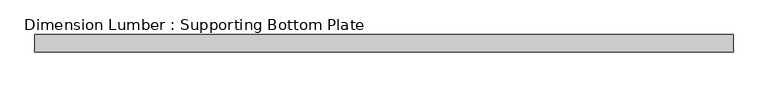
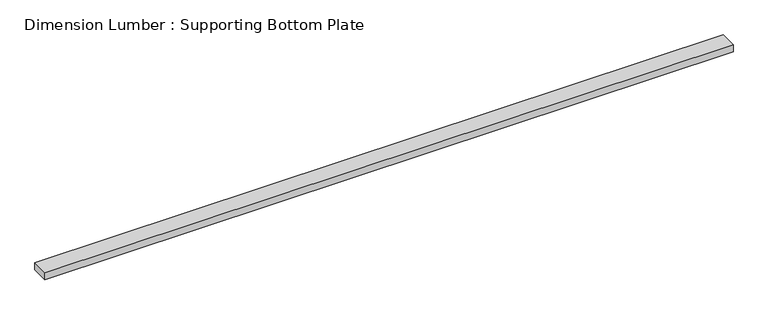
"""IFC4 building model written with IfcOpenShell, lengths in millimetres: beam geometry, Dimension Lumber : Supporting Bottom Plate."""

import ifcopenshell
import ifcopenshell.guid

model = None  # the IFC model being written
_history = None  # IfcOwnerHistory: only IFC2X3 demands one
_inside = {}  # id of a spatial element -> (the spatial element, [elements in it])
_under = {}  # id of a project, library or spatial element -> (it, [spatial elements below it])
_declared = {}  # id of a project -> (the project, [libraries it declares])
_typed = {}  # id of a type object -> (the type object, [elements of that type])
_made_of = {}  # id of a material, layer set ... -> (it, [elements and type objects made of it])


def new_model(schema):
    """Start an empty IFC model of exactly this schema.

    Asked for "IFC4X3", IfcOpenShell would pick the latest addendum, in which some entities
    have other attributes; the version numbers below select the first issue.
    IFC2X3 requires an IfcOwnerHistory on every rooted entity: one is made here for all.
    """
    global model, _history
    if schema == "IFC4X3":
        model = ifcopenshell.file(schema_version=(4, 3, 0, 0))
    else:
        model = ifcopenshell.file(schema=schema)
    _inside.clear()
    _under.clear()
    _declared.clear()
    _typed.clear()
    _made_of.clear()
    _history = None
    if model.schema == "IFC2X3":
        org = make("IfcOrganization", Name="unknown")
        user = make(
            "IfcPersonAndOrganization",
            ThePerson=make("IfcPerson", FamilyName="unknown"),
            TheOrganization=org,
        )
        app = make(
            "IfcApplication",
            ApplicationDeveloper=org,
            Version="unknown",
            ApplicationFullName="unknown",
            ApplicationIdentifier="unknown",
        )
        _history = make(
            "IfcOwnerHistory",
            OwningUser=user,
            OwningApplication=app,
            ChangeAction="ADDED",
            CreationDate=0,
        )
    return model


def make(cls, **values):
    """One entity of the class cls with the attributes given. An attribute that is None is left unset."""
    return model.create_entity(
        cls, **{name: value for name, value in values.items() if value is not None}
    )


def rooted(cls, **values):
    """An entity with a GlobalId (a new one), such as an element, a storey or a relation."""
    return make(cls, GlobalId=ifcopenshell.guid.new(), OwnerHistory=_history, **values)


def si_unit(unit_type, name, prefix=None):
    """IfcSIUnit, for example si_unit("LENGTHUNIT", "METRE", prefix="MILLI")."""
    return make("IfcSIUnit", UnitType=unit_type, Prefix=prefix, Name=name)


def assignment(units):
    """IfcUnitAssignment: the units of a project."""
    return None if units is None else make("IfcUnitAssignment", Units=units)


def point(xyz):
    """IfcCartesianPoint."""
    return None if xyz is None else make("IfcCartesianPoint", Coordinates=xyz)


def direction(xyz):
    """IfcDirection."""
    return None if xyz is None else make("IfcDirection", DirectionRatios=xyz)


def frame(location, z_axis=None, x_axis=None):
    """IfcAxis2Placement3D, a coordinate frame: its origin and axes. An axis left out is left unset."""
    return make(
        "IfcAxis2Placement3D",
        Location=point(location),
        Axis=direction(z_axis),
        RefDirection=direction(x_axis),
    )


def origin():
    """The frame at (0, 0, 0) with its axes left unset."""
    return frame((0.0, 0.0, 0.0))


def place(relative_to, where):
    """IfcLocalPlacement: puts the frame where relative to a parent placement (None: the world)."""
    return make(
        "IfcLocalPlacement", PlacementRelTo=relative_to, RelativePlacement=where
    )


def context(
    kind, dimensions, precision=None, world=None, true_north=None, identifier=None
):
    """IfcGeometricRepresentationContext, for example the 3D "Model" context."""
    return make(
        "IfcGeometricRepresentationContext",
        ContextIdentifier=identifier,
        ContextType=kind,
        CoordinateSpaceDimension=dimensions,
        Precision=precision,
        WorldCoordinateSystem=world,
        TrueNorth=true_north,
    )


def project(units=None, contexts=None):
    """IfcProject with its units and contexts."""
    return rooted(
        "IfcProject",
        Name="project",
        RepresentationContexts=contexts,
        UnitsInContext=assignment(units),
    )


def spatial(cls, under=None, at=None, **own):
    """A site, building, storey or space (cls), placed at a placement, below another one or the project."""
    s = rooted(cls, ObjectPlacement=at, **own)
    if under is not None:
        _under.setdefault(under.id(), (under, []))[1].append(s)
    return s


def polyline(points):
    """IfcPolyline through the points."""
    return make("IfcPolyline", Points=[point(p) for p in points])


def outline(outer, holes=None, kind="AREA"):
    """IfcArbitraryClosedProfileDef: a profile drawn as a closed curve; with holes, ...WithVoids."""
    if holes is None:
        return make("IfcArbitraryClosedProfileDef", ProfileType=kind, OuterCurve=outer)
    return make(
        "IfcArbitraryProfileDefWithVoids",
        ProfileType=kind,
        OuterCurve=outer,
        InnerCurves=holes,
    )


def extrude(swept, where, along, depth):
    """IfcExtrudedAreaSolid: the profile swept, set in the frame where, extruded along a direction by depth."""
    return make(
        "IfcExtrudedAreaSolid",
        SweptArea=swept,
        Position=where,
        ExtrudedDirection=direction(along),
        Depth=depth,
    )


def shape(context_of_items, identifier, shape_type, items):
    """IfcShapeRepresentation: the items that make up one representation, for example the "Body"."""
    return make(
        "IfcShapeRepresentation",
        ContextOfItems=context_of_items,
        RepresentationIdentifier=identifier,
        RepresentationType=shape_type,
        Items=items,
    )


def source(mapping_origin, context_of_items, identifier, shape_type, items):
    """IfcRepresentationMap: a shape defined once, which mapped items show again and again."""
    return make(
        "IfcRepresentationMap",
        MappingOrigin=mapping_origin,
        MappedRepresentation=shape(context_of_items, identifier, shape_type, items),
    )


def transform(
    local_origin,
    x_axis=None,
    y_axis=None,
    z_axis=None,
    scale=None,
    scale2=None,
    scale3=None,
    uniform=True,
):
    """IfcCartesianTransformationOperator3D, or its non-uniform kind. x_axis, y_axis, z_axis: its Axis1, 2, 3."""
    if uniform:
        return make(
            "IfcCartesianTransformationOperator3D",
            Axis1=direction(x_axis),
            Axis2=direction(y_axis),
            LocalOrigin=point(local_origin),
            Scale=scale,
            Axis3=direction(z_axis),
        )
    return make(
        "IfcCartesianTransformationOperator3DnonUniform",
        Axis1=direction(x_axis),
        Axis2=direction(y_axis),
        LocalOrigin=point(local_origin),
        Scale=scale,
        Axis3=direction(z_axis),
        Scale2=scale2,
        Scale3=scale3,
    )


def mapped(mapping_source, mapping_target):
    """IfcMappedItem: shows the shape of a source again, moved by a transform."""
    return make(
        "IfcMappedItem", MappingSource=mapping_source, MappingTarget=mapping_target
    )


def made_of(thing, what):
    """Note that an element or type object is made of a material, layer set ...; save() writes the relation."""
    if what is not None:
        _made_of.setdefault(what.id(), (what, []))[1].append(thing)
    return thing


def element(
    cls,
    number,
    at=None,
    inside=None,
    cuts=None,
    type_object=None,
    material=None,
    context=None,
    identifier="Body",
    shape_type=None,
    held_by="IfcProductDefinitionShape",
    body=None,
    shapes=None,
    **own,
):
    """One element of the class cls, such as IfcWall. Its Tag is "e" and its number.

    at: its placement. inside: the storey or other place that contains it. cuts: it is an
    opening in that element (IfcRelVoidsElement). A single representation is given by context,
    identifier, shape_type and body (its items); several are given by shapes. held_by: the class
    of the entity that holds the representations. save() writes the other relations.
    """
    e = rooted(cls, Tag="e%d" % number, ObjectPlacement=at, **own)
    if body is not None:
        shapes = [shape(context, identifier, shape_type, body)]
    if shapes is not None:
        e.Representation = make(held_by, Representations=shapes)
    if inside is not None:
        _inside.setdefault(inside.id(), (inside, []))[1].append(e)
    if cuts is not None:
        rooted(
            "IfcRelVoidsElement", RelatingBuildingElement=cuts, RelatedOpeningElement=e
        )
    if type_object is not None:
        _typed.setdefault(type_object.id(), (type_object, []))[1].append(e)
    return made_of(e, material)


def aggregate(whole, parts):
    """IfcRelAggregates: a whole, such as a stair, and the parts it consists of."""
    return rooted("IfcRelAggregates", RelatingObject=whole, RelatedObjects=parts)


def save(model, path):
    """Write the relations noted so far, then the file.

    IfcRelAggregates (storeys below a building ...), IfcRelContainedInSpatialStructure (elements
    in a storey), IfcRelDefinesByType, IfcRelAssociatesMaterial and IfcRelDeclares: one each for
    every whole, place, type object, material and project.
    """
    for whole, parts in _under.values():
        aggregate(whole, parts)
    for where, things in _inside.values():
        rooted(
            "IfcRelContainedInSpatialStructure",
            RelatedElements=things,
            RelatingStructure=where,
        )
    for kind, things in _typed.values():
        rooted("IfcRelDefinesByType", RelatedObjects=things, RelatingType=kind)
    for what, things in _made_of.values():
        rooted("IfcRelAssociatesMaterial", RelatedObjects=things, RelatingMaterial=what)
    for by, libraries in _declared.values():
        rooted("IfcRelDeclares", RelatingContext=by, RelatedDefinitions=libraries)
    model.write(path)


def dimension_lumber_supporting_bottom_plate_2ddee0ef(model_context):
    return source(origin(), model_context, "Body", "SweptSolid", [
        extrude(outline(polyline([(1771.65, 44.45), (1771.65, -44.45), (-1768.475, -44.45), (-1768.475, 44.45), (1771.65, 44.45)])), frame((0.0, 0.0, -19.05), z_axis=(0.0, 0.0, 1.0), x_axis=(1.0, 0.0, 0.0)), (0.0, 0.0, 1.0), 38.1),
    ])


if __name__ == "__main__":
    model = new_model("IFC4")
    model_context = context("Model", 3, world=origin())
    ifc_project = project(units=[si_unit("LENGTHUNIT", "METRE", prefix="MILLI")], contexts=[model_context])
    site = spatial("IfcSite", under=ifc_project)
    building = spatial("IfcBuilding", under=site)
    placement = place(None, origin())
    dimension_lumber_supporting_bottom_plate_shape = dimension_lumber_supporting_bottom_plate_2ddee0ef(model_context)
    element("IfcBeam", 1, ObjectType="Dimension Lumber : Supporting Bottom Plate", at=placement, inside=building, context=model_context, shape_type="MappedRepresentation", body=[
        mapped(dimension_lumber_supporting_bottom_plate_shape, transform((0.0, 0.0, 0.0), x_axis=(1.0, 0.0, 0.0), y_axis=(0.0, 1.0, 0.0), z_axis=(0.0, 0.0, 1.0))),
    ])
    save(model, "model.ifc")

# Revit data of these elements
# Type "Dimension Lumber : Supporting Bottom Plate"
#   Assembly Code = "B10"
#   A = 0.0364583 SF
#   Length [instance default] = 5' - 0"
#   b = 0' - 3 1/2"
#   d = 0' - 1 1/2"
#   Structural Material [instance default] = Softwood, Lumber
# Element 1 (IfcBeam, "Dimension Lumber : Supporting Bottom Plate")
#   Structural Material = Douglas Fir #2
#   Materials on its faces: "Douglas Fir #2"
# Materials
#   "Softwood, Lumber": class "Wood", colour RGB 223 192 134, transparency 0, Description = "Pinus Echinata", Cost = 0
#   "Douglas Fir #2": class "Wood", colour RGB 223 192 134, transparency 0, Description = "Pinus Echinata", Cost = 0
